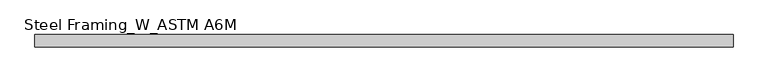
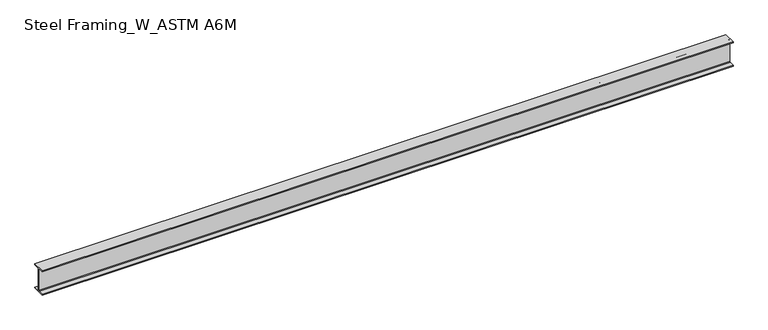
"""IFC4 building model written with IfcOpenShell, lengths in millimetres: beam geometry, Steel Framing_W_ASTM A6M : H_SB_AR_S02_W360x51_B4."""

from ifc_helpers import new_model, si_unit, point, frame, frame_2d, origin, place, context, project, spatial, polyline, circle_curve, trimmed, segment, composite_curve, outline, extrude, source, transform, mapped, element, save


def steel_framing_w_astm_a6m_7a51451f(model_context):
    return source(origin(), model_context, "Body", "SweptSolid", [
        extrude(outline(composite_curve([segment(polyline([(85.5, -166.4), (85.5, -178.0), (-85.5, -178.0), (-85.5, -166.4), (-13.72, -166.4)]), True, "CONTINUOUS"), segment(trimmed(circle_curve(frame_2d((-13.72, -156.3)), 10.1), [point((-13.72, -166.4))], [point((-3.62, -156.3))], True, "CARTESIAN"), True, "CONTINUOUS"), segment(polyline([(-3.62, -156.3), (-3.62, 156.3)]), True, "CONTINUOUS"), segment(trimmed(circle_curve(frame_2d((-13.72, 156.3)), 10.1), [point((-3.62, 156.3))], [point((-13.72, 166.4))], True, "CARTESIAN"), True, "CONTINUOUS"), segment(polyline([(-13.72, 166.4), (-85.5, 166.4), (-85.5, 178.0), (85.5, 178.0), (85.5, 166.4), (13.72, 166.4)]), True, "CONTINUOUS"), segment(trimmed(circle_curve(frame_2d((13.72, 156.3)), 10.1), [point((13.72, 166.4))], [point((3.62, 156.3))], True, "CARTESIAN"), True, "CONTINUOUS"), segment(polyline([(3.62, 156.3), (3.62, -156.3)]), True, "CONTINUOUS"), segment(trimmed(circle_curve(frame_2d((13.72, -156.3)), 10.1), [point((3.62, -156.3))], [point((13.72, -166.4))], True, "CARTESIAN"), True, "CONTINUOUS"), segment(polyline([(13.72, -166.4), (85.5, -166.4)]), True, "CONTINUOUS")], self_intersect=False)), frame((-4901.8, 0.0, 0.0), z_axis=(1.0, 0.0, 0.0), x_axis=(0.0, 1.0, 0.0)), (0.0, 0.0, 1.0), 9619.7),
    ])


if __name__ == "__main__":
    model = new_model("IFC4")
    model_context = context("Model", 3, world=origin())
    ifc_project = project(units=[si_unit("LENGTHUNIT", "METRE", prefix="MILLI")], contexts=[model_context])
    site = spatial("IfcSite", under=ifc_project)
    building = spatial("IfcBuilding", under=site)
    placement = place(None, origin())
    steel_framing_w_astm_a6m_shape = steel_framing_w_astm_a6m_7a51451f(model_context)
    element("IfcBeam", 1, ObjectType="Steel Framing_W_ASTM A6M : H_SB_AR_S02_W360x51_B4", at=placement, inside=building, context=model_context, shape_type="MappedRepresentation", body=[
        mapped(steel_framing_w_astm_a6m_shape, transform((0.0, 0.0, 0.0), x_axis=(1.0, 0.0, 0.0), y_axis=(0.0, 1.0, 0.0), z_axis=(0.0, 0.0, 1.0))),
    ])
    save(model, "model.ifc")

# Revit data of these elements
# Type "Steel Framing_W_ASTM A6M : H_SB_AR_S02_W360x51_B4"
#   Type Mark = "B4"
#   Section Name Key = "W14x34"
#   Width = 17.1 cm
#   Web Thickness = 0.724 cm
#   Web Fillet = 1.01 cm
#   Warping Constant = 287000.0 cm⁶
#   Torsional Moment of Inertia = 23.70 cm⁴
#   Section Area = 64.5 cm²
#   Plastic Modulus weak axis = 174.0 cm³
#   Plastic Modulus strong axis = 895.0 cm³
#   Perimeter = 1.36 m²/m
#   Nominal Weight = 51.00 kgf/m
#   Moment of Inertia weak axis = 970.00 cm⁴
#   Moment of Inertia strong axis = 14200.00 cm⁴
#   Height = 35.6 cm
#   Flange Thickness = 1.16 cm
#   Elastic Modulus weak axis = 113.0 cm³
#   Elastic Modulus strong axis = 796.0 cm³
#   Centroid Vertical = 17.8 cm
#   Centroid Horizontal = 8.55 cm
#   Length [instance default] = 1500 mm
#   Structural Material [instance default] = Steel, 45-345
#   Bolt Spacing = 0
#   Assembly Code = ""
# Element 1 (IfcBeam, "Steel Framing_W_ASTM A6M : H_SB_AR_S02_W360x51_B4")
#   Materials on its faces: "Steel, 45-345"
# Materials
#   "Steel, 45-345": class "Metal", colour RGB 189 187 185, transparency 0, Description = "Steel 345 MPa", Cost = 0
